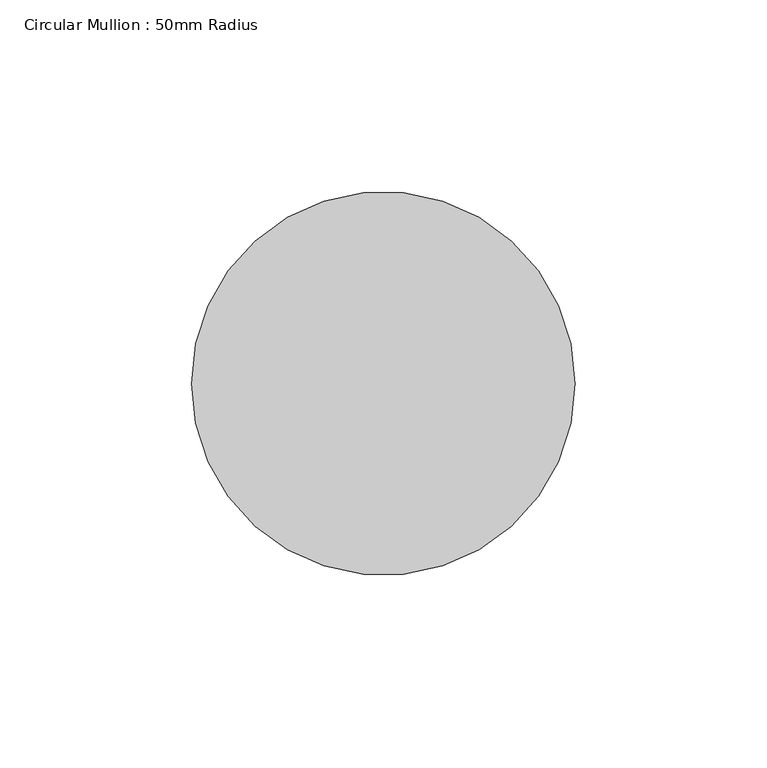
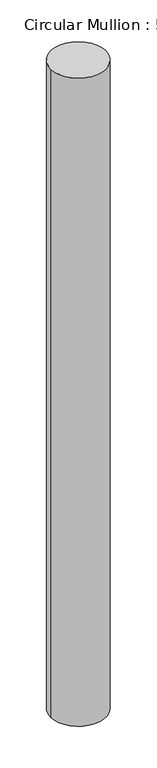
"""IFC4 building model written with IfcOpenShell, lengths in millimetres: member geometry, Circular Mullion : 50mm Radius."""

from ifc_helpers import new_model, si_unit, point, frame, origin, origin_2d, place, context, project, spatial, circle_curve, trimmed, segment, composite_curve, outline, extrude, source, transform, mapped, element, save


def circular_mullion_50mm_radius_6efc73e6(model_context):
    return source(origin(), model_context, "Body", "SweptSolid", [
        extrude(outline(composite_curve([segment(trimmed(circle_curve(origin_2d(), 50.0), [point((50.0, 0.0))], [point((-50.0, 0.0))], False, "CARTESIAN"), True, "CONTINUOUS"), segment(trimmed(circle_curve(origin_2d(), 50.0), [point((-50.0, 0.0))], [point((50.0, 0.0))], False, "CARTESIAN"), True, "CONTINUOUS")], self_intersect=False)), frame((0.0, 0.0, -1238.353404), z_axis=(0.0, 0.0, 1.0), x_axis=(1.0, 0.0, 0.0)), (0.0, 0.0, 1.0), 1238.353404),
    ])


if __name__ == "__main__":
    model = new_model("IFC4")
    model_context = context("Model", 3, world=origin())
    ifc_project = project(units=[si_unit("LENGTHUNIT", "METRE", prefix="MILLI")], contexts=[model_context])
    site = spatial("IfcSite", under=ifc_project)
    building = spatial("IfcBuilding", under=site)
    placement = place(None, origin())
    circular_mullion_50mm_radius_shape = circular_mullion_50mm_radius_6efc73e6(model_context)
    element("IfcMember", 1, ObjectType="Circular Mullion : 50mm Radius", at=placement, inside=building, context=model_context, shape_type="MappedRepresentation", body=[
        mapped(circular_mullion_50mm_radius_shape, transform((0.0, 0.0, 0.0), x_axis=(1.0, 0.0, 0.0), y_axis=(0.0, 1.0, 0.0), z_axis=(0.0, 0.0, 1.0))),
    ])
    save(model, "model.ifc")

# Revit data of these elements
# Type "Circular Mullion : 50mm Radius"
#   built-in parameter 1007350 = 0.164042 (stored number, unit not read)
# Element 1 (IfcMember, "Circular Mullion : 50mm Radius")
#   Materials on its faces: "Aluminium"
# Materials
#   "Aluminium": class "Metal", colour RGB 247 247 247, transparency 0, Description = "Aluminium 6061", Cost = 0
